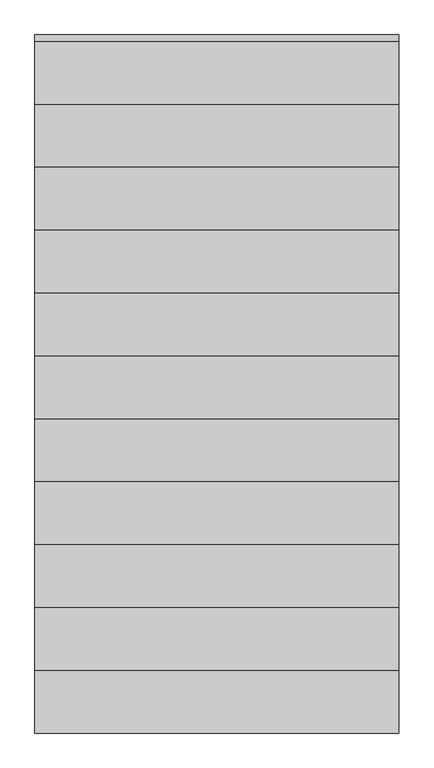
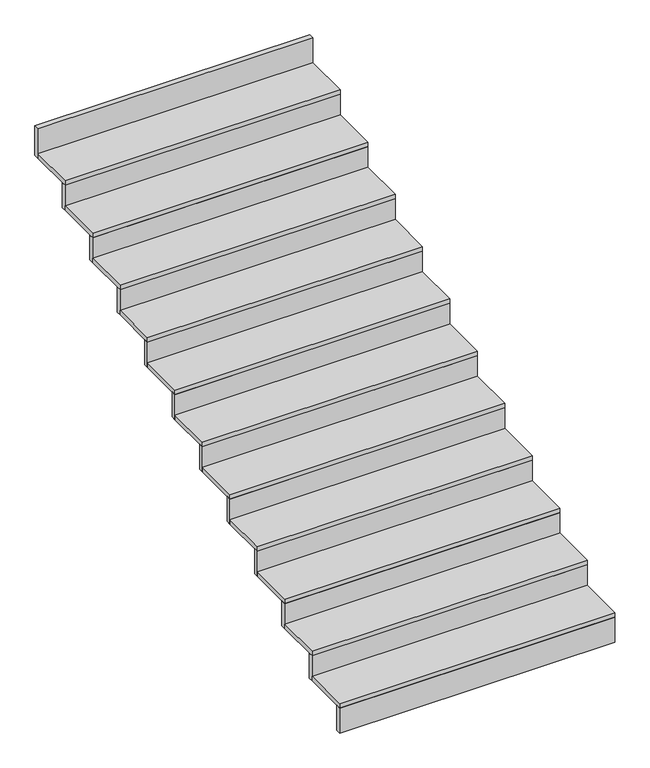
"""IFC4 building model written with IfcOpenShell, lengths in millimetres: stair flight geometry."""

from ifc_helpers import new_model, si_unit, frame, origin, place, context, project, spatial, polyline, outline, extrude, source, transform, mapped, element, save


def stair_flight_ec9a2fb4(model_context):
    return source(origin(), model_context, "Body", "SweptSolid", [
        extrude(outline(polyline([(52810.0, -5570.0), (52810.0, -5600.0), (51075.0, -5600.0), (51075.0, -5570.0), (52810.0, -5570.0)])), frame((0.0, 0.0, 16770.0), z_axis=(0.0, 0.0, 1.0), x_axis=(1.0, 0.0, 0.0)), (0.0, 0.0, 1.0), 166.6666667),
        extrude(outline(polyline([(51075.0, -5300.0), (52810.0, -5300.0), (52810.0, -5600.0), (51075.0, -5600.0), (51075.0, -5300.0)])), frame((0.0, 0.0, 16936.6666667), z_axis=(0.0, 0.0, 1.0), x_axis=(1.0, 0.0, 0.0)), (0.0, 0.0, 1.0), 30.0),
        extrude(outline(polyline([(52810.0, -5270.0), (52810.0, -5300.0), (51075.0, -5300.0), (51075.0, -5270.0), (52810.0, -5270.0)])), frame((0.0, 0.0, 16936.6666667), z_axis=(0.0, 0.0, 1.0), x_axis=(1.0, 0.0, 0.0)), (0.0, 0.0, 1.0), 166.6666667),
        extrude(outline(polyline([(51075.0, -5000.0), (52810.0, -5000.0), (52810.0, -5300.0), (51075.0, -5300.0), (51075.0, -5000.0)])), frame((0.0, 0.0, 17103.3333333), z_axis=(0.0, 0.0, 1.0), x_axis=(1.0, 0.0, 0.0)), (0.0, 0.0, 1.0), 30.0),
        extrude(outline(polyline([(52810.0, -4970.0), (52810.0, -5000.0), (51075.0, -5000.0), (51075.0, -4970.0), (52810.0, -4970.0)])), frame((0.0, 0.0, 17103.3333333), z_axis=(0.0, 0.0, 1.0), x_axis=(1.0, 0.0, 0.0)), (0.0, 0.0, 1.0), 166.6666667),
        extrude(outline(polyline([(51075.0, -4700.0), (52810.0, -4700.0), (52810.0, -5000.0), (51075.0, -5000.0), (51075.0, -4700.0)])), frame((0.0, 0.0, 17270.0), z_axis=(0.0, 0.0, 1.0), x_axis=(1.0, 0.0, 0.0)), (0.0, 0.0, 1.0), 30.0),
        extrude(outline(polyline([(52810.0, -4670.0), (52810.0, -4700.0), (51075.0, -4700.0), (51075.0, -4670.0), (52810.0, -4670.0)])), frame((0.0, 0.0, 17270.0), z_axis=(0.0, 0.0, 1.0), x_axis=(1.0, 0.0, 0.0)), (0.0, 0.0, 1.0), 166.6666667),
        extrude(outline(polyline([(51075.0, -4400.0), (52810.0, -4400.0), (52810.0, -4700.0), (51075.0, -4700.0), (51075.0, -4400.0)])), frame((0.0, 0.0, 17436.6666667), z_axis=(0.0, 0.0, 1.0), x_axis=(1.0, 0.0, 0.0)), (0.0, 0.0, 1.0), 30.0),
        extrude(outline(polyline([(52810.0, -4370.0), (52810.0, -4400.0), (51075.0, -4400.0), (51075.0, -4370.0), (52810.0, -4370.0)])), frame((0.0, 0.0, 17436.6666667), z_axis=(0.0, 0.0, 1.0), x_axis=(1.0, 0.0, 0.0)), (0.0, 0.0, 1.0), 166.6666667),
        extrude(outline(polyline([(51075.0, -4100.0), (52810.0, -4100.0), (52810.0, -4400.0), (51075.0, -4400.0), (51075.0, -4100.0)])), frame((0.0, 0.0, 17603.3333333), z_axis=(0.0, 0.0, 1.0), x_axis=(1.0, 0.0, 0.0)), (0.0, 0.0, 1.0), 30.0),
        extrude(outline(polyline([(52810.0, -4070.0), (52810.0, -4100.0), (51075.0, -4100.0), (51075.0, -4070.0), (52810.0, -4070.0)])), frame((0.0, 0.0, 17603.3333333), z_axis=(0.0, 0.0, 1.0), x_axis=(1.0, 0.0, 0.0)), (0.0, 0.0, 1.0), 166.6666667),
        extrude(outline(polyline([(51075.0, -3800.0), (52810.0, -3800.0), (52810.0, -4100.0), (51075.0, -4100.0), (51075.0, -3800.0)])), frame((0.0, 0.0, 17770.0), z_axis=(0.0, 0.0, 1.0), x_axis=(1.0, 0.0, 0.0)), (0.0, 0.0, 1.0), 30.0),
        extrude(outline(polyline([(52810.0, -3770.0), (52810.0, -3800.0), (51075.0, -3800.0), (51075.0, -3770.0), (52810.0, -3770.0)])), frame((0.0, 0.0, 17770.0), z_axis=(0.0, 0.0, 1.0), x_axis=(1.0, 0.0, 0.0)), (0.0, 0.0, 1.0), 166.6666667),
        extrude(outline(polyline([(51075.0, -3500.0), (52810.0, -3500.0), (52810.0, -3800.0), (51075.0, -3800.0), (51075.0, -3500.0)])), frame((0.0, 0.0, 17936.6666667), z_axis=(0.0, 0.0, 1.0), x_axis=(1.0, 0.0, 0.0)), (0.0, 0.0, 1.0), 30.0),
        extrude(outline(polyline([(52810.0, -3470.0), (52810.0, -3500.0), (51075.0, -3500.0), (51075.0, -3470.0), (52810.0, -3470.0)])), frame((0.0, 0.0, 17936.6666667), z_axis=(0.0, 0.0, 1.0), x_axis=(1.0, 0.0, 0.0)), (0.0, 0.0, 1.0), 166.6666667),
        extrude(outline(polyline([(51075.0, -3200.0), (52810.0, -3200.0), (52810.0, -3500.0), (51075.0, -3500.0), (51075.0, -3200.0)])), frame((0.0, 0.0, 18103.3333333), z_axis=(0.0, 0.0, 1.0), x_axis=(1.0, 0.0, 0.0)), (0.0, 0.0, 1.0), 30.0),
        extrude(outline(polyline([(52810.0, -3170.0), (52810.0, -3200.0), (51075.0, -3200.0), (51075.0, -3170.0), (52810.0, -3170.0)])), frame((0.0, 0.0, 18103.3333333), z_axis=(0.0, 0.0, 1.0), x_axis=(1.0, 0.0, 0.0)), (0.0, 0.0, 1.0), 166.6666667),
        extrude(outline(polyline([(51075.0, -2900.0), (52810.0, -2900.0), (52810.0, -3200.0), (51075.0, -3200.0), (51075.0, -2900.0)])), frame((0.0, 0.0, 18270.0), z_axis=(0.0, 0.0, 1.0), x_axis=(1.0, 0.0, 0.0)), (0.0, 0.0, 1.0), 30.0),
        extrude(outline(polyline([(52810.0, -2870.0), (52810.0, -2900.0), (51075.0, -2900.0), (51075.0, -2870.0), (52810.0, -2870.0)])), frame((0.0, 0.0, 18270.0), z_axis=(0.0, 0.0, 1.0), x_axis=(1.0, 0.0, 0.0)), (0.0, 0.0, 1.0), 166.6666667),
        extrude(outline(polyline([(51075.0, -2600.0), (52810.0, -2600.0), (52810.0, -2900.0), (51075.0, -2900.0), (51075.0, -2600.0)])), frame((0.0, 0.0, 18436.6666667), z_axis=(0.0, 0.0, 1.0), x_axis=(1.0, 0.0, 0.0)), (0.0, 0.0, 1.0), 30.0),
        extrude(outline(polyline([(52810.0, -2570.0), (52810.0, -2600.0), (51075.0, -2600.0), (51075.0, -2570.0), (52810.0, -2570.0)])), frame((0.0, 0.0, 18436.6666667), z_axis=(0.0, 0.0, 1.0), x_axis=(1.0, 0.0, 0.0)), (0.0, 0.0, 1.0), 166.6666667),
        extrude(outline(polyline([(52810.0, -2270.0), (52810.0, -2300.0), (51075.0, -2300.0), (51075.0, -2270.0), (52810.0, -2270.0)])), frame((0.0, 0.0, 18603.3333333), z_axis=(0.0, 0.0, 1.0), x_axis=(1.0, 0.0, 0.0)), (0.0, 0.0, 1.0), 196.6666667),
        extrude(outline(polyline([(51075.0, -2300.0), (52810.0, -2300.0), (52810.0, -2600.0), (51075.0, -2600.0), (51075.0, -2300.0)])), frame((0.0, 0.0, 18603.3333333), z_axis=(0.0, 0.0, 1.0), x_axis=(1.0, 0.0, 0.0)), (0.0, 0.0, 1.0), 30.0),
    ])


if __name__ == "__main__":
    model = new_model("IFC4")
    model_context = context("Model", 3, world=origin())
    ifc_project = project(units=[si_unit("LENGTHUNIT", "METRE", prefix="MILLI")], contexts=[model_context])
    site = spatial("IfcSite", under=ifc_project)
    building = spatial("IfcBuilding", under=site)
    placement = place(None, origin())
    stair_flight_shape = stair_flight_ec9a2fb4(model_context)
    element("IfcStairFlight", 1, at=placement, inside=building, context=model_context, shape_type="MappedRepresentation", body=[
        mapped(stair_flight_shape, transform((0.0, 0.0, 0.0), x_axis=(1.0, 0.0, 0.0), y_axis=(0.0, 1.0, 0.0), z_axis=(0.0, 0.0, 1.0))),
    ])
    save(model, "model.ifc")

# Revit data of these elements
# Element 1 (IfcStairFlight)
#   Materials on its faces: "00_Finish_Deco Tile"
# Materials
#   "00_Finish_Deco Tile": class "Finish", colour RGB 245 245 245, transparency 0, Description = "Ceramic Tile", Cost = 0
